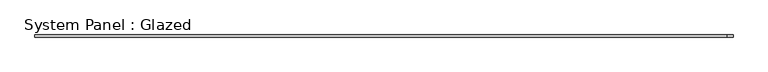
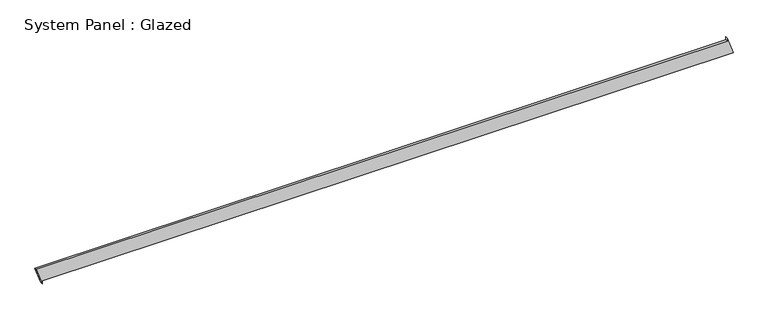
"""IFC4 building model written with IfcOpenShell, lengths in millimetres: plate geometry, System Panel : Glazed."""

from ifc_helpers import new_model, si_unit, frame, origin, place, context, project, spatial, polyline, outline, extrude, source, transform, mapped, element, save


def system_panel_glazed_81bebace(model_context):
    return source(origin(), model_context, "Body", "SweptSolid", [
        extrude(outline(polyline([(0.0, -3958.4984909), (35.3553391, -3958.4984909), (35.3553391, 4028.1402063), (235.3994701, 3958.60512), (200.0441311, 3958.6053171), (199.9996015, -4028.1402063), (0.0, -3958.4984909)])), frame((0.0, -49.5, 0.0), z_axis=(0.0, 1.0, 0.0), x_axis=(0.0, 0.0, 1.0)), (0.0, 0.0, 1.0), 25.0),
    ])


if __name__ == "__main__":
    model = new_model("IFC4")
    model_context = context("Model", 3, world=origin())
    ifc_project = project(units=[si_unit("LENGTHUNIT", "METRE", prefix="MILLI")], contexts=[model_context])
    site = spatial("IfcSite", under=ifc_project)
    building = spatial("IfcBuilding", under=site)
    placement = place(None, origin())
    system_panel_glazed_shape = system_panel_glazed_81bebace(model_context)
    element("IfcPlate", 1, ObjectType="System Panel : Glazed", at=placement, inside=building, context=model_context, shape_type="MappedRepresentation", body=[
        mapped(system_panel_glazed_shape, transform((0.0, 0.0, 0.0), x_axis=(1.0, 0.0, 0.0), y_axis=(0.0, 1.0, 0.0), z_axis=(0.0, 0.0, 1.0))),
    ])
    save(model, "model.ifc")

# Revit data of these elements
# Element 1 (IfcPlate, "System Panel : Glazed")
#   Materials on its faces: "Glass"
# Materials
#   "Glass": class "Glass", colour RGB 218 227 224, transparency 0.85, Description = "Soda Lime Glass", Cost = 0
